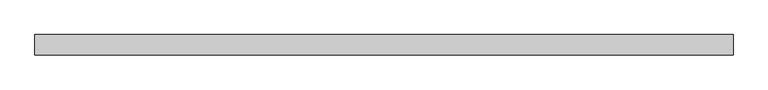
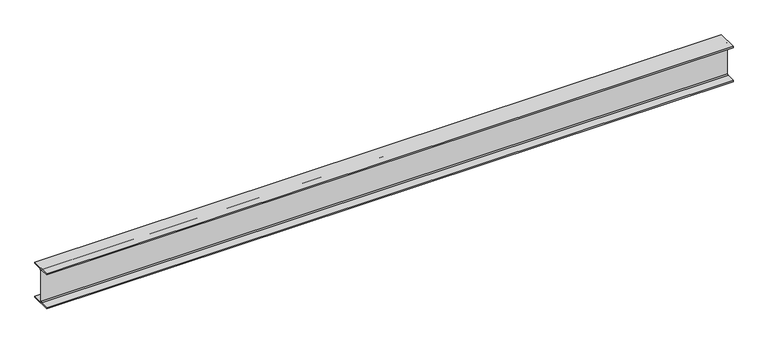
"""IFC4 building model written with IfcOpenShell, lengths in millimetres: beam geometry, Steel Beam_H-KSD3502 : H_SB_ASB_H-200x200x8x12."""

from ifc_helpers import new_model, si_unit, point, frame, frame_2d, origin, place, context, project, spatial, polyline, circle_curve, trimmed, segment, composite_curve, outline, extrude, source, transform, mapped, element, save


def beam_c67ea157(model_context):
    return source(origin(), model_context, "Body", "SweptSolid", [
        extrude(outline(composite_curve([segment(polyline([(82.5, -141.5), (82.5, -151.7), (-82.5, -151.7), (-82.5, -141.5), (-11.9, -141.5)]), True, "CONTINUOUS"), segment(trimmed(circle_curve(frame_2d((-11.9, -132.6)), 8.9), [point((-11.9, -141.5))], [point((-3.0, -132.6))], True, "CARTESIAN"), True, "CONTINUOUS"), segment(polyline([(-3.0, -132.6), (-3.0, 132.6)]), True, "CONTINUOUS"), segment(trimmed(circle_curve(frame_2d((-11.9, 132.6)), 8.9), [point((-3.0, 132.6))], [point((-11.9, 141.5))], True, "CARTESIAN"), True, "CONTINUOUS"), segment(polyline([(-11.9, 141.5), (-82.5, 141.5), (-82.5, 151.7), (82.5, 151.7), (82.5, 141.5), (11.9, 141.5)]), True, "CONTINUOUS"), segment(trimmed(circle_curve(frame_2d((11.9, 132.6)), 8.9), [point((11.9, 141.5))], [point((3.0, 132.6))], True, "CARTESIAN"), True, "CONTINUOUS"), segment(polyline([(3.0, 132.6), (3.0, -132.6)]), True, "CONTINUOUS"), segment(trimmed(circle_curve(frame_2d((11.9, -132.6)), 8.9), [point((3.0, -132.6))], [point((11.9, -141.5))], True, "CARTESIAN"), True, "CONTINUOUS"), segment(polyline([(11.9, -141.5), (82.5, -141.5)]), True, "CONTINUOUS")], self_intersect=False)), frame((-2934.658354, 0.0, 0.0), z_axis=(1.0, 0.0, 0.0), x_axis=(0.0, 1.0, 0.0)), (0.0, 0.0, 1.0), 5622.4398071),
    ])


if __name__ == "__main__":
    model = new_model("IFC4")
    model_context = context("Model", 3, world=origin())
    ifc_project = project(units=[si_unit("LENGTHUNIT", "METRE", prefix="MILLI")], contexts=[model_context])
    site = spatial("IfcSite", under=ifc_project)
    building = spatial("IfcBuilding", under=site)
    placement = place(None, origin())
    beam_shape = beam_c67ea157(model_context)
    element("IfcBeam", 1, ObjectType="Steel Beam_H-KSD3502 : H_SB_ASB_H-200x200x8x12", at=placement, inside=building, context=model_context, shape_type="MappedRepresentation", body=[
        mapped(beam_shape, transform((0.0, 0.0, 0.0), x_axis=(1.0, 0.0, 0.0), y_axis=(0.0, 1.0, 0.0), z_axis=(0.0, 0.0, 1.0))),
    ])
    save(model, "model.ifc")

# Revit data of these elements
# Type "Steel Beam_H-KSD3502 : H_SB_ASB_H-200x200x8x12"
#   Width = 20.0 cm
#   Web Thickness = 0.8 cm
#   Web Fillet = 1.3 cm
#   Warping Constant = 141376.0 cm⁶
#   Torsional Moment of Inertia = 26.2485 cm⁴
#   Torsional Modulus = 1.0 cm³
#   Section Area = 63.53 cm²
#   Plastic Modulus weak axis = 244.0 cm³
#   Plastic Modulus strong axis = 525.0 cm³
#   Perimeter = 1.16 m²/m
#   Nominal Weight = 49.90 kgf/m
#   Moment of Inertia weak axis = 1600.00 cm⁴
#   Moment of Inertia strong axis = 4720.00 cm⁴
#   Height = 20.0 cm
#   Flange Thickness = 1.2 cm
#   Elastic Modulus weak axis = 160.0 cm³
#   Elastic Modulus strong axis = 472.0 cm³
#   Centroid Vertical = 10.0 cm
#   Centroid Horizontal = 10.0 cm
#   Length [instance default] = 1.5240 m
#   Structural Material [instance default] = Steel, 45-345
#   Assembly Code = ""
# Element 1 (IfcBeam, "Steel Beam_H-KSD3502 : H_SB_ASB_H-200x200x8x12")
#   Structural Material = none
# Materials
#   "Steel, 45-345": class "Metal", colour RGB 189 187 185, transparency 0, Description = "Steel 345 MPa", Cost = 0
